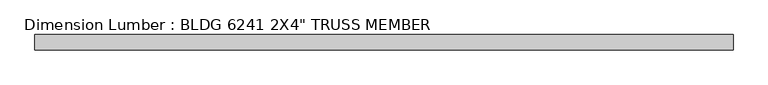
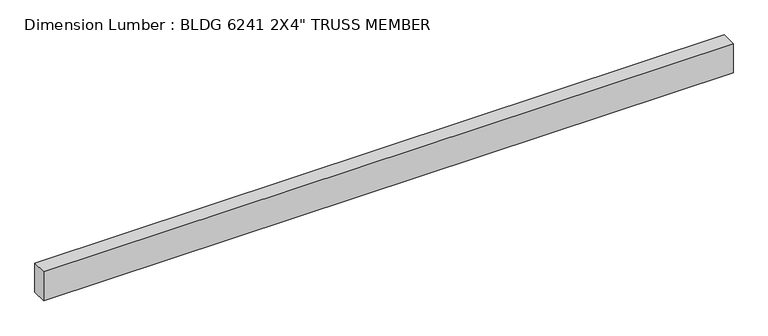
"""IFC4 building model written with IfcOpenShell, lengths in millimetres: beam geometry."""

from ifc_helpers import new_model, si_unit, frame, origin, place, context, project, spatial, polyline, outline, extrude, source, transform, mapped, element, save


def beam_0b80d38c(model_context):
    return source(origin(), model_context, "Body", "SweptSolid", [
        extrude(outline(polyline([(1143.0, 25.4), (1143.0, -25.4), (-1143.0, -25.4), (-1143.0, 25.4), (1143.0, 25.4)])), frame((0.0, 0.0, -50.8), z_axis=(0.0, 0.0, 1.0), x_axis=(1.0, 0.0, 0.0)), (0.0, 0.0, 1.0), 101.6),
    ])


if __name__ == "__main__":
    model = new_model("IFC4")
    model_context = context("Model", 3, world=origin())
    ifc_project = project(units=[si_unit("LENGTHUNIT", "METRE", prefix="MILLI")], contexts=[model_context])
    site = spatial("IfcSite", under=ifc_project)
    building = spatial("IfcBuilding", under=site)
    placement = place(None, origin())
    beam_shape = beam_0b80d38c(model_context)
    element("IfcBeam", 1, ObjectType="Dimension Lumber : BLDG 6241 2X4\" TRUSS MEMBER", at=placement, inside=building, context=model_context, shape_type="MappedRepresentation", body=[
        mapped(beam_shape, transform((0.0, 0.0, 0.0), x_axis=(1.0, 0.0, 0.0), y_axis=(0.0, 1.0, 0.0), z_axis=(0.0, 0.0, 1.0))),
    ])
    save(model, "model.ifc")

# Revit data of these elements
# Type "Dimension Lumber : BLDG 6241 2X4\" TRUSS MEMBER"
#   Assembly Code = "B10"
#   A = 0.273472 SF
#   Length [instance default] = 5' - 0"
#   b = 0' - 2"
#   d = 0' - 4"
#   Structural Material [instance default] = Softwood, Lumber
# Element 1 (IfcBeam, "Dimension Lumber : BLDG 6241 2X4\" TRUSS MEMBER")
#   Materials on its faces: "Softwood, Lumber"
# Materials
#   "Softwood, Lumber": class "Wood", colour RGB 223 192 134, transparency 0, Description = "Pinus Echinata", Cost = 0
